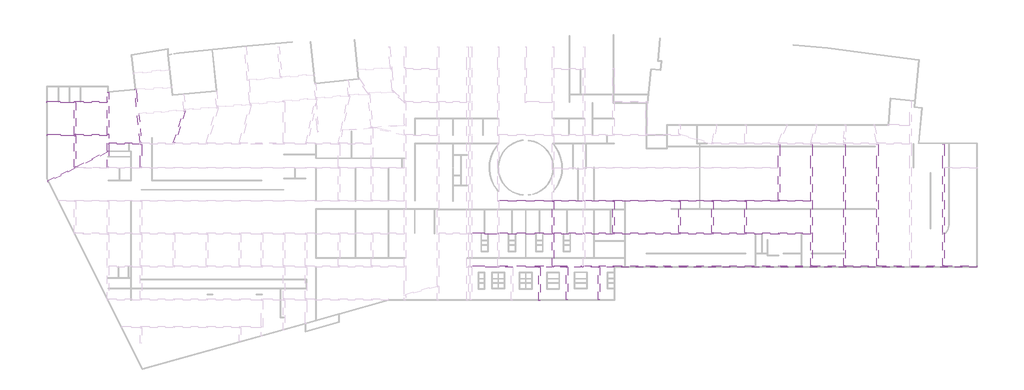
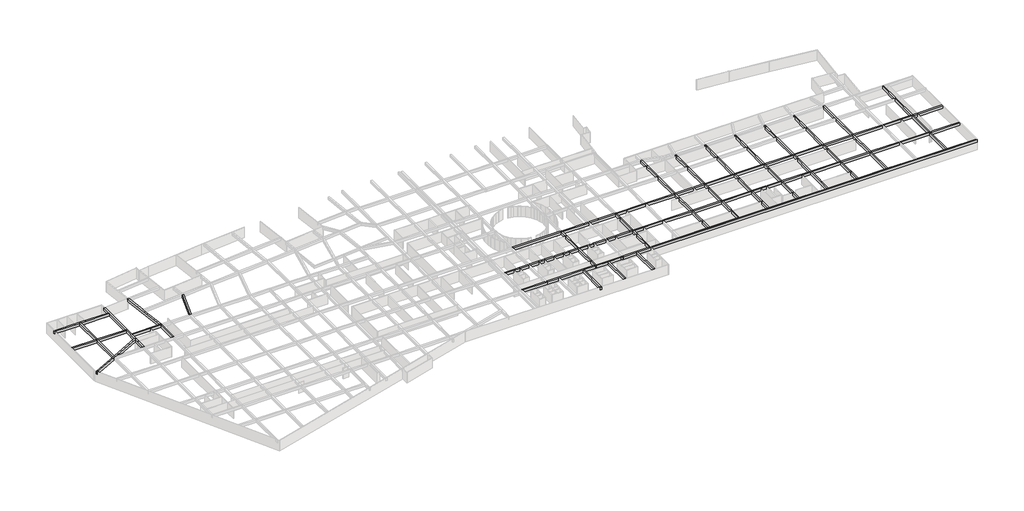
# One storey, part 6 of 8: 38 beams.
"""IFC4 building model written with IfcOpenShell, lengths in millimetres."""

from ifc_helpers import new_model, si_unit, frame, origin, place, context, project, spatial, polyline, outline, extrude, faceted_brep, element, save

model = new_model("IFC4")

# Units and contexts
model_context = context("Model", 3, world=origin())
ifc_project = project(units=[si_unit("LENGTHUNIT", "METRE", prefix="MILLI")], contexts=[model_context])

# Site, building, storey
site = spatial("IfcSite", under=ifc_project)
building = spatial("IfcBuilding", under=site)
storey = spatial("IfcBuildingStorey", under=building, Name="户型图", Elevation=0.0)

# Beams
placement = place(None, origin())
element("IfcBeam", 1, ObjectType="混凝土 - 矩形梁 : KL_beam", at=placement, inside=storey, context=model_context, shape_type="Brep", body=[
    faceted_brep([(544553.8653576, 12938.6264904, 3300.0), (544153.8653576, 12938.6264904, 3300.0), (544153.8653576, 6738.6264904, 3300.0), (544153.8653576, 6338.6264904, 3300.0), (544153.8653576, -2261.3735096, 3300.0), (544153.8653576, -2661.3735096, 3300.0), (544153.8653576, -11261.3735096, 3300.0), (544153.8653576, -11661.3735096, 3300.0), (544153.8653576, -20261.3735096, 3300.0), (544553.8653576, -20261.3735096, 3300.0), (544553.8653576, -11661.3735096, 3300.0), (544553.8653576, -11261.3735096, 3300.0), (544553.8653576, -2661.3735096, 3300.0), (544553.8653576, -2261.3735096, 3300.0), (544553.8653576, 6338.6264904, 3300.0), (544553.8653576, 6738.6264904, 3300.0), (544153.8653576, 12938.6264904, 2500.0), (544153.8653576, 6738.6264904, 2500.0), (544153.8653576, 6338.6264904, 2500.0), (544153.8653576, -2261.3735096, 2500.0), (544153.8653576, -2661.3735096, 2500.0), (544153.8653576, -11261.3735096, 2500.0), (544153.8653576, -11661.3735096, 2500.0), (544153.8653576, -20261.3735096, 2500.0), (544553.8653576, 12938.6264904, 2500.0), (544553.8653576, 6738.6264904, 2500.0), (544553.8653576, 6338.6264904, 2500.0), (544553.8653576, -2261.3735096, 2500.0), (544553.8653576, -2661.3735096, 2500.0), (544553.8653576, -11261.3735096, 2500.0), (544553.8653576, -11661.3735096, 2500.0), (544553.8653576, -20261.3735096, 2500.0)], [[[0, 1, 2, 3, 4, 5, 6, 7, 8, 9, 10, 11, 12, 13, 14, 15]], [[1, 16, 17, 18, 19, 20, 21, 22, 23, 8, 7, 6, 5, 4, 3, 2]], [[16, 24, 25, 26, 27, 28, 29, 30, 31, 23, 22, 21, 20, 19, 18, 17]], [[24, 0, 15, 14, 13, 12, 11, 10, 9, 31, 30, 29, 28, 27, 26, 25]], [[1, 0, 24, 16]], [[9, 8, 23, 31]]]),
])
element("IfcBeam", 2, ObjectType="混凝土 - 矩形梁 : KL_beam", at=placement, inside=storey, context=model_context, shape_type="Brep", body=[
    faceted_brep([(526553.8653576, 12938.6264904, 3300.0), (526153.8653576, 12938.6264904, 3300.0), (526153.8653576, 6738.6264904, 3300.0), (526153.8653576, 6338.6264904, 3300.0), (526153.8653576, -2261.3735096, 3300.0), (526153.8653576, -2661.3735096, 3300.0), (526153.8653576, -11261.3735096, 3300.0), (526153.8653576, -11661.3735096, 3300.0), (526153.8653576, -20261.3735096, 3300.0), (526553.8653576, -20261.3735096, 3300.0), (526553.8653576, -11661.3735096, 3300.0), (526553.8653576, -11261.3735096, 3300.0), (526553.8653576, -2661.3735096, 3300.0), (526553.8653576, -2261.3735096, 3300.0), (526553.8653576, 6338.6264904, 3300.0), (526553.8653576, 6738.6264904, 3300.0), (526153.8653576, 12938.6264904, 2500.0), (526153.8653576, 6738.6264904, 2500.0), (526153.8653576, 6338.6264904, 2500.0), (526153.8653576, -2261.3735096, 2500.0), (526153.8653576, -2661.3735096, 2500.0), (526153.8653576, -11261.3735096, 2500.0), (526153.8653576, -11661.3735096, 2500.0), (526153.8653576, -20261.3735096, 2500.0), (526553.8653576, 12938.6264904, 2500.0), (526553.8653576, 6738.6264904, 2500.0), (526553.8653576, 6338.6264904, 2500.0), (526553.8653576, -2261.3735096, 2500.0), (526553.8653576, -2661.3735096, 2500.0), (526553.8653576, -11261.3735096, 2500.0), (526553.8653576, -11661.3735096, 2500.0), (526553.8653576, -20261.3735096, 2500.0)], [[[0, 1, 2, 3, 4, 5, 6, 7, 8, 9, 10, 11, 12, 13, 14, 15]], [[1, 16, 17, 18, 19, 20, 21, 22, 23, 8, 7, 6, 5, 4, 3, 2]], [[16, 24, 25, 26, 27, 28, 29, 30, 31, 23, 22, 21, 20, 19, 18, 17]], [[24, 0, 15, 14, 13, 12, 11, 10, 9, 31, 30, 29, 28, 27, 26, 25]], [[1, 0, 24, 16]], [[9, 8, 23, 31]]]),
])
element("IfcBeam", 3, ObjectType="混凝土 - 矩形梁 : KL_beam", at=placement, inside=storey, context=model_context, shape_type="Brep", body=[
    faceted_brep([(517553.8653576, 12938.6264904, 3300.0), (517153.8653576, 12938.6264904, 3300.0), (517153.8653576, 6738.6264904, 3300.0), (517153.8653576, 6338.6264904, 3300.0), (517153.8653576, -2261.3735096, 3300.0), (517153.8653576, -2661.3735096, 3300.0), (517153.8653576, -11261.3735096, 3300.0), (517153.8653576, -11661.3735096, 3300.0), (517153.8653576, -20261.3735096, 3300.0), (517553.8653576, -20261.3735096, 3300.0), (517553.8653576, -11661.3735096, 3300.0), (517553.8653576, -11261.3735096, 3300.0), (517553.8653576, -2661.3735096, 3300.0), (517553.8653576, -2261.3735096, 3300.0), (517553.8653576, 6338.6264904, 3300.0), (517553.8653576, 6738.6264904, 3300.0), (517553.8653576, 12938.6264904, 2500.0), (517553.8653576, -20261.3735096, 2500.0), (517553.8653576, -11661.3735096, 2500.0), (517553.8653576, -11261.3735096, 2500.0), (517553.8653576, -2661.3735096, 2500.0), (517553.8653576, -2261.3735096, 2500.0), (517553.8653576, 6338.6264904, 2500.0), (517553.8653576, 6738.6264904, 2500.0), (517153.8653576, 12938.6264904, 2500.0), (517153.8653576, -20261.3735096, 2500.0), (517153.8653576, -11661.3735096, 2500.0), (517153.8653576, -11261.3735096, 2500.0), (517153.8653576, -2661.3735096, 2500.0), (517153.8653576, -2261.3735096, 2500.0), (517153.8653576, 6338.6264904, 2500.0), (517153.8653576, 6738.6264904, 2500.0)], [[[0, 1, 2, 3, 4, 5, 6, 7, 8, 9, 10, 11, 12, 13, 14, 15]], [[16, 0, 15, 14, 13, 12, 11, 10, 9, 17, 18, 19, 20, 21, 22, 23]], [[24, 16, 23, 22, 21, 20, 19, 18, 17, 25, 26, 27, 28, 29, 30, 31]], [[1, 24, 31, 30, 29, 28, 27, 26, 25, 8, 7, 6, 5, 4, 3, 2]], [[1, 0, 16, 24]], [[9, 8, 25, 17]]]),
])
element("IfcBeam", 4, ObjectType="混凝土 - 矩形梁 : KL_beam", at=placement, inside=storey, context=model_context, shape_type="Brep", body=[
    faceted_brep([(508553.8653576, 12938.6264904, 3300.0), (508153.8653576, 12938.6264904, 3300.0), (508153.8653576, 6738.6264904, 3300.0), (508153.8653576, 6338.6264904, 3300.0), (508153.8653576, -2261.3735096, 3300.0), (508153.8653576, -2661.3735096, 3300.0), (508153.8653576, -11261.3735096, 3300.0), (508153.8653576, -11661.3735096, 3300.0), (508153.8653576, -20261.3735096, 3300.0), (508553.8653576, -20261.3735096, 3300.0), (508553.8653576, -11661.3735096, 3300.0), (508553.8653576, -11261.3735096, 3300.0), (508553.8653576, -2661.3735096, 3300.0), (508553.8653576, -2261.3735096, 3300.0), (508553.8653576, 6338.6264904, 3300.0), (508553.8653576, 6738.6264904, 3300.0), (508153.8653576, 12938.6264904, 2500.0), (508153.8653576, 6738.6264904, 2500.0), (508153.8653576, 6338.6264904, 2500.0), (508153.8653576, -2261.3735096, 2500.0), (508153.8653576, -2661.3735096, 2500.0), (508153.8653576, -11261.3735096, 2500.0), (508153.8653576, -11661.3735096, 2500.0), (508153.8653576, -20261.3735096, 2500.0), (508553.8653576, 12938.6264904, 2500.0), (508553.8653576, 6738.6264904, 2500.0), (508553.8653576, 6338.6264904, 2500.0), (508553.8653576, -2261.3735096, 2500.0), (508553.8653576, -2661.3735096, 2500.0), (508553.8653576, -11261.3735096, 2500.0), (508553.8653576, -11661.3735096, 2500.0), (508553.8653576, -20261.3735096, 2500.0)], [[[0, 1, 2, 3, 4, 5, 6, 7, 8, 9, 10, 11, 12, 13, 14, 15]], [[1, 16, 17, 18, 19, 20, 21, 22, 23, 8, 7, 6, 5, 4, 3, 2]], [[16, 24, 25, 26, 27, 28, 29, 30, 31, 23, 22, 21, 20, 19, 18, 17]], [[24, 0, 15, 14, 13, 12, 11, 10, 9, 31, 30, 29, 28, 27, 26, 25]], [[1, 0, 24, 16]], [[9, 8, 23, 31]]]),
])
element("IfcBeam", 5, ObjectType="混凝土 - 矩形梁 : KL_beam", at=placement, inside=storey, context=model_context, shape_type="Brep", body=[
    faceted_brep([(553518.3052108, -2661.3735096, 3300.0), (553518.3052108, -2661.3735096, 2500.0), (553518.3052108, -2261.3735096, 2500.0), (553518.3052108, -2261.3735096, 3300.0), (544553.8653576, -2661.3735096, 3300.0), (544553.8653576, -2261.3735096, 3300.0), (544553.8653576, -2261.3735096, 2500.0), (544553.8653576, -2661.3735096, 2500.0)], [[[0, 1, 2, 3]], [[4, 5, 6, 7]], [[0, 3, 5, 4]], [[3, 2, 6, 5]], [[2, 1, 7, 6]], [[1, 0, 4, 7]]]),
    faceted_brep([(544153.8653576, -2661.3735096, 3300.0), (544153.8653576, -2261.3735096, 3300.0), (535553.8653576, -2261.3735096, 3300.0), (535553.8653576, -2661.3735096, 3300.0), (544153.8653576, -2261.3735096, 2500.0), (535553.8653576, -2261.3735096, 2500.0), (544153.8653576, -2661.3735096, 2500.0), (535553.8653576, -2661.3735096, 2500.0)], [[[0, 1, 2, 3]], [[1, 4, 5, 2]], [[4, 6, 7, 5]], [[6, 0, 3, 7]], [[1, 0, 6, 4]], [[3, 2, 5, 7]]]),
    faceted_brep([(535153.8653576, -2261.3735096, 3300.0), (535153.8653576, -2661.3735096, 3300.0), (535153.8653576, -2661.3735096, 2500.0), (535153.8653576, -2261.3735096, 2500.0), (526553.8653576, -2661.3735096, 3300.0), (526553.8653576, -2261.3735096, 3300.0), (526553.8653576, -2261.3735096, 2500.0), (526553.8653576, -2661.3735096, 2500.0)], [[[0, 1, 2, 3]], [[4, 5, 6, 7]], [[1, 0, 5, 4]], [[0, 3, 6, 5]], [[3, 2, 7, 6]], [[2, 1, 4, 7]]]),
    faceted_brep([(526153.8653576, -2661.3735096, 3300.0), (526153.8653576, -2261.3735096, 3300.0), (517553.8653576, -2261.3735096, 3300.0), (517553.8653576, -2661.3735096, 3300.0), (526153.8653576, -2261.3735096, 2500.0), (517553.8653576, -2261.3735096, 2500.0), (526153.8653576, -2661.3735096, 2500.0), (517553.8653576, -2661.3735096, 2500.0)], [[[0, 1, 2, 3]], [[1, 4, 5, 2]], [[4, 6, 7, 5]], [[6, 0, 3, 7]], [[1, 0, 6, 4]], [[3, 2, 5, 7]]]),
    faceted_brep([(517153.8653576, -2261.3735096, 3300.0), (517153.8653576, -2661.3735096, 3300.0), (517153.8653576, -2661.3735096, 2500.0), (517153.8653576, -2261.3735096, 2500.0), (508553.8653576, -2661.3735096, 3300.0), (508553.8653576, -2261.3735096, 3300.0), (508553.8653576, -2261.3735096, 2500.0), (508553.8653576, -2661.3735096, 2500.0)], [[[0, 1, 2, 3]], [[4, 5, 6, 7]], [[1, 0, 5, 4]], [[0, 3, 6, 5]], [[3, 2, 7, 6]], [[2, 1, 4, 7]]]),
    faceted_brep([(508153.8653576, -2261.3735096, 3300.0), (508153.8653576, -2661.3735096, 3300.0), (508153.8653576, -2661.3735096, 2500.0), (508153.8653576, -2261.3735096, 2500.0), (499653.8653576, -2261.3735096, 3300.0), (499253.8653576, -2261.3735096, 3300.0), (490553.8653576, -2261.3735096, 3300.0), (490153.8653576, -2261.3735096, 3300.0), (481553.8653576, -2261.3735096, 3300.0), (481153.8653576, -2261.3735096, 3300.0), (472553.8653576, -2261.3735096, 3300.0), (472153.8653576, -2261.3735096, 3300.0), (463553.8653576, -2261.3735096, 3300.0), (463153.8653576, -2261.3735096, 3300.0), (454553.8653576, -2261.3735096, 3300.0), (454153.8653576, -2261.3735096, 3300.0), (446453.8653576, -2261.3735096, 3300.0), (446453.8653576, -2661.3735096, 3300.0), (454153.8653576, -2661.3735096, 3300.0), (454553.8653576, -2661.3735096, 3300.0), (463153.8653576, -2661.3735096, 3300.0), (463553.8653576, -2661.3735096, 3300.0), (472153.8653576, -2661.3735096, 3300.0), (472553.8653576, -2661.3735096, 3300.0), (481153.8653576, -2661.3735096, 3300.0), (481553.8653576, -2661.3735096, 3300.0), (490153.8653576, -2661.3735096, 3300.0), (490553.8653576, -2661.3735096, 3300.0), (499253.8653576, -2661.3735096, 3300.0), (499653.8653576, -2661.3735096, 3300.0), (499653.8653576, -2261.3735096, 2500.0), (499253.8653576, -2261.3735096, 2500.0), (490553.8653576, -2261.3735096, 2500.0), (490153.8653576, -2261.3735096, 2500.0), (481553.8653576, -2261.3735096, 2500.0), (481153.8653576, -2261.3735096, 2500.0), (472553.8653576, -2261.3735096, 2500.0), (472153.8653576, -2261.3735096, 2500.0), (463553.8653576, -2261.3735096, 2500.0), (463153.8653576, -2261.3735096, 2500.0), (454553.8653576, -2261.3735096, 2500.0), (454153.8653576, -2261.3735096, 2500.0), (446453.8653576, -2261.3735096, 2500.0), (499653.8653576, -2661.3735096, 2500.0), (499253.8653576, -2661.3735096, 2500.0), (490553.8653576, -2661.3735096, 2500.0), (490153.8653576, -2661.3735096, 2500.0), (481553.8653576, -2661.3735096, 2500.0), (481153.8653576, -2661.3735096, 2500.0), (472553.8653576, -2661.3735096, 2500.0), (472153.8653576, -2661.3735096, 2500.0), (463553.8653576, -2661.3735096, 2500.0), (463153.8653576, -2661.3735096, 2500.0), (454553.8653576, -2661.3735096, 2500.0), (454153.8653576, -2661.3735096, 2500.0), (446453.8653576, -2661.3735096, 2500.0)], [[[0, 1, 2, 3]], [[1, 0, 4, 5, 6, 7, 8, 9, 10, 11, 12, 13, 14, 15, 16, 17, 18, 19, 20, 21, 22, 23, 24, 25, 26, 27, 28, 29]], [[0, 3, 30, 31, 32, 33, 34, 35, 36, 37, 38, 39, 40, 41, 42, 16, 15, 14, 13, 12, 11, 10, 9, 8, 7, 6, 5, 4]], [[3, 2, 43, 44, 45, 46, 47, 48, 49, 50, 51, 52, 53, 54, 55, 42, 41, 40, 39, 38, 37, 36, 35, 34, 33, 32, 31, 30]], [[2, 1, 29, 28, 27, 26, 25, 24, 23, 22, 21, 20, 19, 18, 17, 55, 54, 53, 52, 51, 50, 49, 48, 47, 46, 45, 44, 43]], [[17, 16, 42, 55]]]),
])
element("IfcBeam", 6, ObjectType="混凝土 - 矩形梁 : KL_beam", at=placement, inside=storey, context=model_context, shape_type="Brep", body=[
    faceted_brep([(553518.3052108, -11661.3735096, 3300.0), (553518.3052108, -11661.3735096, 2500.0), (553518.3052108, -11261.3735096, 2500.0), (553518.3052108, -11261.3735096, 3300.0), (544553.8653576, -11661.3735096, 3300.0), (544553.8653576, -11261.3735096, 3300.0), (544553.8653576, -11261.3735096, 2500.0), (544553.8653576, -11661.3735096, 2500.0)], [[[0, 1, 2, 3]], [[4, 5, 6, 7]], [[0, 3, 5, 4]], [[3, 2, 6, 5]], [[2, 1, 7, 6]], [[1, 0, 4, 7]]]),
    faceted_brep([(544153.8653576, -11661.3735096, 3300.0), (544153.8653576, -11261.3735096, 3300.0), (535553.8653576, -11261.3735096, 3300.0), (535553.8653576, -11661.3735096, 3300.0), (544153.8653576, -11261.3735096, 2500.0), (535553.8653576, -11261.3735096, 2500.0), (544153.8653576, -11661.3735096, 2500.0), (535553.8653576, -11661.3735096, 2500.0)], [[[0, 1, 2, 3]], [[1, 4, 5, 2]], [[4, 6, 7, 5]], [[6, 0, 3, 7]], [[1, 0, 6, 4]], [[3, 2, 5, 7]]]),
    faceted_brep([(535153.8653576, -11261.3735096, 3300.0), (535153.8653576, -11661.3735096, 3300.0), (535153.8653576, -11661.3735096, 2500.0), (535153.8653576, -11261.3735096, 2500.0), (526553.8653576, -11661.3735096, 3300.0), (526553.8653576, -11261.3735096, 3300.0), (526553.8653576, -11261.3735096, 2500.0), (526553.8653576, -11661.3735096, 2500.0)], [[[0, 1, 2, 3]], [[4, 5, 6, 7]], [[1, 0, 5, 4]], [[0, 3, 6, 5]], [[3, 2, 7, 6]], [[2, 1, 4, 7]]]),
    faceted_brep([(526153.8653576, -11661.3735096, 3300.0), (526153.8653576, -11261.3735096, 3300.0), (517553.8653576, -11261.3735096, 3300.0), (517553.8653576, -11661.3735096, 3300.0), (526153.8653576, -11261.3735096, 2500.0), (517553.8653576, -11261.3735096, 2500.0), (526153.8653576, -11661.3735096, 2500.0), (517553.8653576, -11661.3735096, 2500.0)], [[[0, 1, 2, 3]], [[1, 4, 5, 2]], [[4, 6, 7, 5]], [[6, 0, 3, 7]], [[1, 0, 6, 4]], [[3, 2, 5, 7]]]),
    faceted_brep([(517153.8653576, -11261.3735096, 3300.0), (517153.8653576, -11661.3735096, 3300.0), (517153.8653576, -11661.3735096, 2500.0), (517153.8653576, -11261.3735096, 2500.0), (508553.8653576, -11661.3735096, 3300.0), (508553.8653576, -11261.3735096, 3300.0), (508553.8653576, -11261.3735096, 2500.0), (508553.8653576, -11661.3735096, 2500.0)], [[[0, 1, 2, 3]], [[4, 5, 6, 7]], [[1, 0, 5, 4]], [[0, 3, 6, 5]], [[3, 2, 7, 6]], [[2, 1, 4, 7]]]),
    faceted_brep([(508153.8653576, -11261.3735096, 3300.0), (508153.8653576, -11661.3735096, 3300.0), (508153.8653576, -11661.3735096, 2500.0), (508153.8653576, -11261.3735096, 2500.0), (499653.8653576, -11261.3735096, 3300.0), (499253.8653576, -11261.3735096, 3300.0), (490553.8653576, -11261.3735096, 3300.0), (490153.8653576, -11261.3735096, 3300.0), (481553.8653576, -11261.3735096, 3300.0), (481153.8653576, -11261.3735096, 3300.0), (472553.8653576, -11261.3735096, 3300.0), (472153.8653576, -11261.3735096, 3300.0), (463553.8653576, -11261.3735096, 3300.0), (463153.8653576, -11261.3735096, 3300.0), (454553.8653576, -11261.3735096, 3300.0), (454153.8653576, -11261.3735096, 3300.0), (446453.8653576, -11261.3735096, 3300.0), (446453.8653576, -11661.3735096, 3300.0), (454153.8653576, -11661.3735096, 3300.0), (454553.8653576, -11661.3735096, 3300.0), (463153.8653576, -11661.3735096, 3300.0), (463553.8653576, -11661.3735096, 3300.0), (472153.8653576, -11661.3735096, 3300.0), (472553.8653576, -11661.3735096, 3300.0), (481153.8653576, -11661.3735096, 3300.0), (481553.8653576, -11661.3735096, 3300.0), (490153.8653576, -11661.3735096, 3300.0), (490553.8653576, -11661.3735096, 3300.0), (499253.8653576, -11661.3735096, 3300.0), (499653.8653576, -11661.3735096, 3300.0), (499653.8653576, -11261.3735096, 2500.0), (499253.8653576, -11261.3735096, 2500.0), (490553.8653576, -11261.3735096, 2500.0), (490153.8653576, -11261.3735096, 2500.0), (481553.8653576, -11261.3735096, 2500.0), (481153.8653576, -11261.3735096, 2500.0), (472553.8653576, -11261.3735096, 2500.0), (472153.8653576, -11261.3735096, 2500.0), (463553.8653576, -11261.3735096, 2500.0), (463153.8653576, -11261.3735096, 2500.0), (454553.8653576, -11261.3735096, 2500.0), (454153.8653576, -11261.3735096, 2500.0), (446453.8653576, -11261.3735096, 2500.0), (499653.8653576, -11661.3735096, 2500.0), (499253.8653576, -11661.3735096, 2500.0), (490553.8653576, -11661.3735096, 2500.0), (490153.8653576, -11661.3735096, 2500.0), (481553.8653576, -11661.3735096, 2500.0), (481153.8653576, -11661.3735096, 2500.0), (472553.8653576, -11661.3735096, 2500.0), (472153.8653576, -11661.3735096, 2500.0), (463553.8653576, -11661.3735096, 2500.0), (463153.8653576, -11661.3735096, 2500.0), (454553.8653576, -11661.3735096, 2500.0), (454153.8653576, -11661.3735096, 2500.0), (446453.8653576, -11661.3735096, 2500.0)], [[[0, 1, 2, 3]], [[1, 0, 4, 5, 6, 7, 8, 9, 10, 11, 12, 13, 14, 15, 16, 17, 18, 19, 20, 21, 22, 23, 24, 25, 26, 27, 28, 29]], [[0, 3, 30, 31, 32, 33, 34, 35, 36, 37, 38, 39, 40, 41, 42, 16, 15, 14, 13, 12, 11, 10, 9, 8, 7, 6, 5, 4]], [[3, 2, 43, 44, 45, 46, 47, 48, 49, 50, 51, 52, 53, 54, 55, 42, 41, 40, 39, 38, 37, 36, 35, 34, 33, 32, 31, 30]], [[2, 1, 29, 28, 27, 26, 25, 24, 23, 22, 21, 20, 19, 18, 17, 55, 54, 53, 52, 51, 50, 49, 48, 47, 46, 45, 44, 43]], [[17, 16, 42, 55]]]),
])
element("IfcBeam", 7, ObjectType="混凝土 - 矩形梁 : KL_beam", at=placement, inside=storey, context=model_context, shape_type="Brep", body=[
    faceted_brep([(553453.8653576, -20261.3735096, 3300.0), (553453.8653576, -20661.3735096, 3300.0), (553453.8653576, -20661.3735096, 2500.0), (553453.8653576, -20261.3735096, 2500.0), (544553.8653576, -20261.3735096, 3300.0), (544153.8653576, -20261.3735096, 3300.0), (535553.8653576, -20261.3735096, 3300.0), (535153.8653576, -20261.3735096, 3300.0), (526553.8653576, -20261.3735096, 3300.0), (526153.8653576, -20261.3735096, 3300.0), (517553.8653576, -20261.3735096, 3300.0), (517153.8653576, -20261.3735096, 3300.0), (508553.8653576, -20261.3735096, 3300.0), (508153.8653576, -20261.3735096, 3300.0), (499653.8653576, -20261.3735096, 3300.0), (499253.8653576, -20261.3735096, 3300.0), (490553.8653576, -20261.3735096, 3300.0), (490153.8653576, -20261.3735096, 3300.0), (481553.8653576, -20261.3735096, 3300.0), (481153.8653576, -20261.3735096, 3300.0), (472553.8653576, -20261.3735096, 3300.0), (472153.8653576, -20261.3735096, 3300.0), (463553.8653576, -20261.3735096, 3300.0), (463153.8653576, -20261.3735096, 3300.0), (454553.8653576, -20261.3735096, 3300.0), (454153.8653576, -20261.3735096, 3300.0), (446453.8653576, -20261.3735096, 3300.0), (446053.8653576, -20261.3735096, 3300.0), (446053.8653576, -20661.3735096, 3300.0), (450103.8653576, -20661.3735096, 3300.0), (450503.8653576, -20661.3735096, 3300.0), (446053.8653576, -20661.3735096, 2500.0), (450103.8653576, -20661.3735096, 2500.0), (450503.8653576, -20661.3735096, 2500.0), (446053.8653576, -20261.3735096, 2500.0), (446453.8653576, -20261.3735096, 2500.0), (454153.8653576, -20261.3735096, 2500.0), (454553.8653576, -20261.3735096, 2500.0), (463153.8653576, -20261.3735096, 2500.0), (463553.8653576, -20261.3735096, 2500.0), (472153.8653576, -20261.3735096, 2500.0), (472553.8653576, -20261.3735096, 2500.0), (481153.8653576, -20261.3735096, 2500.0), (481553.8653576, -20261.3735096, 2500.0), (490153.8653576, -20261.3735096, 2500.0), (490553.8653576, -20261.3735096, 2500.0), (499253.8653576, -20261.3735096, 2500.0), (499653.8653576, -20261.3735096, 2500.0), (508153.8653576, -20261.3735096, 2500.0), (508553.8653576, -20261.3735096, 2500.0), (517153.8653576, -20261.3735096, 2500.0), (517553.8653576, -20261.3735096, 2500.0), (526153.8653576, -20261.3735096, 2500.0), (526553.8653576, -20261.3735096, 2500.0), (535153.8653576, -20261.3735096, 2500.0), (535553.8653576, -20261.3735096, 2500.0), (544153.8653576, -20261.3735096, 2500.0), (544553.8653576, -20261.3735096, 2500.0)], [[[0, 1, 2, 3]], [[1, 0, 4, 5, 6, 7, 8, 9, 10, 11, 12, 13, 14, 15, 16, 17, 18, 19, 20, 21, 22, 23, 24, 25, 26, 27, 28, 29, 30]], [[2, 1, 30, 29, 28, 31, 32, 33]], [[3, 2, 33, 32, 31, 34, 35, 36, 37, 38, 39, 40, 41, 42, 43, 44, 45, 46, 47, 48, 49, 50, 51, 52, 53, 54, 55, 56, 57]], [[0, 3, 57, 56, 55, 54, 53, 52, 51, 50, 49, 48, 47, 46, 45, 44, 43, 42, 41, 40, 39, 38, 37, 36, 35, 34, 27, 26, 25, 24, 23, 22, 21, 20, 19, 18, 17, 16, 15, 14, 13, 12, 11, 10, 9, 8, 7, 6, 5, 4]], [[28, 27, 34, 31]]]),
])
element("IfcBeam", 8, ObjectType="混凝土 - 矩形梁 : KL_beam", at=placement, inside=storey, context=model_context, shape_type="Brep", body=[
    faceted_brep([(472153.8653576, -20261.3735096, 3300.0), (472553.8653576, -20261.3735096, 3300.0), (472553.8653576, -11661.3735096, 3300.0), (472153.8653576, -11661.3735096, 3300.0), (472153.8653576, -20261.3735096, 2500.0), (472153.8653576, -11661.3735096, 2500.0), (472553.8653576, -20261.3735096, 2500.0), (472553.8653576, -11661.3735096, 2500.0)], [[[0, 1, 2, 3]], [[4, 0, 3, 5]], [[6, 4, 5, 7]], [[1, 6, 7, 2]], [[1, 0, 4, 6]], [[3, 2, 7, 5]]]),
    faceted_brep([(472153.8653576, 15338.6264904, 3300.0), (472553.8653576, 15338.6264904, 3300.0), (472553.8653576, 15338.6264904, 2500.0), (472153.8653576, 15338.6264904, 2500.0), (472553.8653576, 6738.6264904, 3300.0), (472153.8653576, 6738.6264904, 3300.0), (472153.8653576, 6738.6264904, 2500.0), (472553.8653576, 6738.6264904, 2500.0), (472553.8653576, 15278.3041611, 3300.0), (472553.8653576, 15278.3041611, 2500.0)], [[[0, 1, 2, 3]], [[4, 5, 6, 7]], [[1, 0, 5, 4, 8]], [[0, 3, 6, 5]], [[3, 2, 9, 7, 6]], [[2, 1, 8, 4, 7, 9]]]),
    faceted_brep([(472553.8653576, -2261.3735096, 3300.0), (472153.8653576, -2261.3735096, 3300.0), (472153.8653576, -2261.3735096, 2500.0), (472553.8653576, -2261.3735096, 2500.0), (472553.8653576, 6338.6264904, 3300.0), (472153.8653576, 6338.6264904, 3300.0), (472153.8653576, 6338.6264904, 2500.0), (472553.8653576, 6338.6264904, 2500.0)], [[[0, 1, 2, 3]], [[1, 0, 4, 5]], [[2, 1, 5, 6]], [[3, 2, 6, 7]], [[0, 3, 7, 4]], [[5, 4, 7, 6]]]),
    faceted_brep([(472153.8653576, -2661.3735096, 3300.0), (472553.8653576, -2661.3735096, 3300.0), (472553.8653576, -2661.3735096, 2500.0), (472153.8653576, -2661.3735096, 2500.0), (472553.8653576, -11261.3735096, 3300.0), (472153.8653576, -11261.3735096, 3300.0), (472153.8653576, -11261.3735096, 2500.0), (472553.8653576, -11261.3735096, 2500.0)], [[[0, 1, 2, 3]], [[4, 5, 6, 7]], [[1, 0, 5, 4]], [[0, 3, 6, 5]], [[3, 2, 7, 6]], [[2, 1, 4, 7]]]),
])
element("IfcBeam", 9, ObjectType="混凝土 - 矩形梁 : KL_beam", at=placement, inside=storey, context=model_context, shape_type="SweptSolid", body=[
    extrude(outline(polyline([(481153.8653576, 12938.6264904), (481553.8653576, 12938.6264904), (481553.8653576, 6738.6264904), (481153.8653576, 6738.6264904), (481153.8653576, 12938.6264904)])), frame((0.0, 0.0, 2500.0), z_axis=(0.0, 0.0, 1.0), x_axis=(1.0, 0.0, 0.0)), (0.0, 0.0, 1.0), 800.0),
    extrude(outline(polyline([(481553.8653576, -20261.3735096), (481153.8653576, -20261.3735096), (481153.8653576, -11661.3735096), (481553.8653576, -11661.3735096), (481553.8653576, -20261.3735096)])), frame((0.0, 0.0, 2500.0), z_axis=(0.0, 0.0, 1.0), x_axis=(1.0, 0.0, 0.0)), (0.0, 0.0, 1.0), 800.0),
    extrude(outline(polyline([(481553.8653576, -2261.3735096), (481153.8653576, -2261.3735096), (481153.8653576, 6338.6264904), (481553.8653576, 6338.6264904), (481553.8653576, -2261.3735096)])), frame((0.0, 0.0, 2500.0), z_axis=(0.0, 0.0, 1.0), x_axis=(1.0, 0.0, 0.0)), (0.0, 0.0, 1.0), 800.0),
    extrude(outline(polyline([(481153.8653576, -2661.3735096), (481553.8653576, -2661.3735096), (481553.8653576, -11261.3735096), (481153.8653576, -11261.3735096), (481153.8653576, -2661.3735096)])), frame((0.0, 0.0, 2500.0), z_axis=(0.0, 0.0, 1.0), x_axis=(1.0, 0.0, 0.0)), (0.0, 0.0, 1.0), 800.0),
])
element("IfcBeam", 10, ObjectType="混凝土 - 矩形梁 : KL_beam", at=placement, inside=storey, context=model_context, shape_type="SweptSolid", body=[
    extrude(outline(polyline([(490553.8653576, -20261.3735096), (490153.8653576, -20261.3735096), (490153.8653576, -11661.3735096), (490553.8653576, -11661.3735096), (490553.8653576, -20261.3735096)])), frame((0.0, 0.0, 2500.0), z_axis=(0.0, 0.0, 1.0), x_axis=(1.0, 0.0, 0.0)), (0.0, 0.0, 1.0), 800.0),
    extrude(outline(polyline([(490153.8653576, 12938.6264904), (490553.8653576, 12938.6264904), (490553.8653576, 6738.6264904), (490153.8653576, 6738.6264904), (490153.8653576, 12938.6264904)])), frame((0.0, 0.0, 2500.0), z_axis=(0.0, 0.0, 1.0), x_axis=(1.0, 0.0, 0.0)), (0.0, 0.0, 1.0), 800.0),
    extrude(outline(polyline([(490553.8653576, -2261.3735096), (490153.8653576, -2261.3735096), (490153.8653576, 6338.6264904), (490553.8653576, 6338.6264904), (490553.8653576, -2261.3735096)])), frame((0.0, 0.0, 2500.0), z_axis=(0.0, 0.0, 1.0), x_axis=(1.0, 0.0, 0.0)), (0.0, 0.0, 1.0), 800.0),
    extrude(outline(polyline([(490153.8653576, -2661.3735096), (490553.8653576, -2661.3735096), (490553.8653576, -11261.3735096), (490153.8653576, -11261.3735096), (490153.8653576, -2661.3735096)])), frame((0.0, 0.0, 2500.0), z_axis=(0.0, 0.0, 1.0), x_axis=(1.0, 0.0, 0.0)), (0.0, 0.0, 1.0), 800.0),
])
element("IfcBeam", 11, ObjectType="混凝土 - 矩形梁 : KL_beam", at=placement, inside=storey, context=model_context, shape_type="Brep", body=[
    faceted_brep([(499653.8653576, 12938.6264904, 3300.0), (499253.8653576, 12938.6264904, 3300.0), (499253.8653576, 6738.6264904, 3300.0), (499253.8653576, 6338.6264904, 3300.0), (499253.8653576, -2261.3735096, 3300.0), (499653.8653576, -2261.3735096, 3300.0), (499653.8653576, 6338.6264904, 3300.0), (499653.8653576, 6738.6264904, 3300.0), (499653.8653576, 12938.6264904, 2500.0), (499653.8653576, -2261.3735096, 2500.0), (499653.8653576, 6338.6264904, 2500.0), (499653.8653576, 6738.6264904, 2500.0), (499253.8653576, 12938.6264904, 2500.0), (499253.8653576, -2261.3735096, 2500.0), (499253.8653576, 6338.6264904, 2500.0), (499253.8653576, 6738.6264904, 2500.0)], [[[0, 1, 2, 3, 4, 5, 6, 7]], [[8, 0, 7, 6, 5, 9, 10, 11]], [[12, 8, 11, 10, 9, 13, 14, 15]], [[1, 12, 15, 14, 13, 4, 3, 2]], [[1, 0, 8, 12]], [[5, 4, 13, 9]]]),
    faceted_brep([(499653.8653576, -20261.3735096, 3300.0), (499253.8653576, -20261.3735096, 3300.0), (499253.8653576, -20261.3735096, 2500.0), (499653.8653576, -20261.3735096, 2500.0), (499253.8653576, -11661.3735096, 3300.0), (499653.8653576, -11661.3735096, 3300.0), (499653.8653576, -11661.3735096, 2500.0), (499253.8653576, -11661.3735096, 2500.0)], [[[0, 1, 2, 3]], [[4, 5, 6, 7]], [[1, 0, 5, 4]], [[0, 3, 6, 5]], [[3, 2, 7, 6]], [[2, 1, 4, 7]]]),
    faceted_brep([(499253.8653576, -2661.3735096, 3300.0), (499653.8653576, -2661.3735096, 3300.0), (499653.8653576, -2661.3735096, 2500.0), (499253.8653576, -2661.3735096, 2500.0), (499253.8653576, -11261.3735096, 3300.0), (499653.8653576, -11261.3735096, 3300.0), (499653.8653576, -11261.3735096, 2500.0), (499253.8653576, -11261.3735096, 2500.0)], [[[0, 1, 2, 3]], [[1, 0, 4, 5]], [[2, 1, 5, 6]], [[3, 2, 6, 7]], [[0, 3, 7, 4]], [[5, 4, 7, 6]]]),
])
element("IfcBeam", 12, ObjectType="混凝土 - 矩形梁 : KL_beam", at=placement, inside=storey, context=model_context, shape_type="SweptSolid", body=[
    extrude(outline(polyline([(454553.8653576, -20261.3735096), (454153.8653576, -20261.3735096), (454153.8653576, -11661.3735096), (454553.8653576, -11661.3735096), (454553.8653576, -20261.3735096)])), frame((0.0, 0.0, 2500.0), z_axis=(0.0, 0.0, 1.0), x_axis=(1.0, 0.0, 0.0)), (0.0, 0.0, 1.0), 800.0),
    extrude(outline(polyline([(454153.8653576, -2661.3735096), (454553.8653576, -2661.3735096), (454553.8653576, -11261.3735096), (454153.8653576, -11261.3735096), (454153.8653576, -2661.3735096)])), frame((0.0, 0.0, 2500.0), z_axis=(0.0, 0.0, 1.0), x_axis=(1.0, 0.0, 0.0)), (0.0, 0.0, 1.0), 800.0),
])
element("IfcBeam", 13, ObjectType="混凝土 - 矩形梁 : KL_beam", at=placement, inside=storey, context=model_context, shape_type="SweptSolid", body=[
    extrude(outline(polyline([(325153.8653576, 12938.6264904), (325553.8653576, 12938.6264904), (325553.8653576, 6738.6264904), (325153.8653576, 6738.6264904), (325153.8653576, 12938.6264904)])), frame((0.0, 0.0, 2500.0), z_axis=(0.0, 0.0, 1.0), x_axis=(1.0, 0.0, 0.0)), (0.0, 0.0, 1.0), 800.0),
])
element("IfcBeam", 14, ObjectType="混凝土 - 矩形梁 : KL_beam", at=placement, inside=storey, context=model_context, shape_type="Brep", body=[
    faceted_brep([(316553.8653576, 15738.6264904, 3300.0), (316153.8653576, 15738.6264904, 3300.0), (316153.8653576, 15338.6264904, 3300.0), (316153.8653576, 11162.2332882, 3300.0), (316153.8653576, 10715.0196927, 3300.0), (316153.8653576, 6738.6264904, 3300.0), (316553.8653576, 6738.6264904, 3300.0), (316553.8653576, 12938.6264904, 3300.0), (316553.8653576, 13338.6264904, 3300.0), (316553.8653576, 15738.6264904, 2500.0), (316553.8653576, 6738.6264904, 2500.0), (316553.8653576, 12938.6264904, 2500.0), (316553.8653576, 13338.6264904, 2500.0), (316153.8653576, 15738.6264904, 2500.0), (316153.8653576, 6738.6264904, 2500.0), (316153.8653576, 10715.0196927, 2500.0), (316153.8653576, 11162.2332882, 2500.0), (316153.8653576, 15338.6264904, 2500.0)], [[[0, 1, 2, 3, 4, 5, 6, 7, 8]], [[9, 0, 8, 7, 6, 10, 11, 12]], [[13, 9, 12, 11, 10, 14, 15, 16, 17]], [[1, 13, 17, 16, 15, 14, 5, 4, 3, 2]], [[6, 5, 14, 10]], [[1, 0, 9, 13]]]),
])
element("IfcBeam", 15, ObjectType="混凝土 - 矩形梁 : KL_beam", at=placement, inside=storey, context=model_context, shape_type="Brep", body=[
    faceted_brep([(307153.8653576, 15738.6264904, 3300.0), (307153.8653576, 15338.6264904, 3300.0), (307553.8653576, 15338.6264904, 3300.0), (316153.8653576, 15338.6264904, 3300.0), (316153.8653576, 15738.6264904, 3300.0), (307553.8653576, 15738.6264904, 3300.0), (307153.8653576, 15738.6264904, 2500.0), (316153.8653576, 15738.6264904, 2500.0), (307553.8653576, 15738.6264904, 2500.0), (307153.8653576, 15338.6264904, 2500.0), (316153.8653576, 15338.6264904, 2500.0), (307553.8653576, 15338.6264904, 2500.0)], [[[0, 1, 2, 3, 4, 5]], [[6, 0, 5, 4, 7, 8]], [[9, 6, 8, 7, 10, 11]], [[1, 9, 11, 10, 3, 2]], [[4, 3, 10, 7]], [[1, 0, 6, 9]]]),
])
element("IfcBeam", 16, ObjectType="混凝土 - 矩形梁 : KL_beam", at=placement, inside=storey, context=model_context, shape_type="Brep", body=[
    faceted_brep([(307553.8653576, 24738.6264904, 3300.0), (307153.8653576, 24738.6264904, 3300.0), (307153.8653576, 24338.6264904, 3300.0), (307153.8653576, 15738.6264904, 3300.0), (307553.8653576, 15738.6264904, 3300.0), (307553.8653576, 24338.6264904, 3300.0), (307553.8653576, 24738.6264904, 2500.0), (307553.8653576, 15738.6264904, 2500.0), (307553.8653576, 24338.6264904, 2500.0), (307153.8653576, 24738.6264904, 2500.0), (307153.8653576, 15738.6264904, 2500.0), (307153.8653576, 24338.6264904, 2500.0)], [[[0, 1, 2, 3, 4, 5]], [[6, 0, 5, 4, 7, 8]], [[9, 6, 8, 7, 10, 11]], [[1, 9, 11, 10, 3, 2]], [[4, 3, 10, 7]], [[1, 0, 6, 9]]]),
])
element("IfcBeam", 17, ObjectType="混凝土 - 矩形梁 : KL_beam", at=placement, inside=storey, context=model_context, shape_type="SweptSolid", body=[
    extrude(outline(polyline([(299553.8653576, 24338.6264904), (299553.8653576, 24738.6264904), (307153.8653576, 24738.6264904), (307153.8653576, 24338.6264904), (299553.8653576, 24338.6264904)])), frame((0.0, 0.0, 2500.0), z_axis=(0.0, 0.0, 1.0), x_axis=(1.0, 0.0, 0.0)), (0.0, 0.0, 1.0), 800.0),
])
element("IfcBeam", 18, ObjectType="混凝土 - 矩形梁 : KL_beam", at=placement, inside=storey, context=model_context, shape_type="SweptSolid", body=[
    extrude(outline(polyline([(299703.8653576, 15338.6264904), (299703.8653576, 15738.6264904), (307153.8653576, 15738.6264904), (307153.8653576, 15338.6264904), (299703.8653576, 15338.6264904)])), frame((0.0, 0.0, 2500.0), z_axis=(0.0, 0.0, 1.0), x_axis=(1.0, 0.0, 0.0)), (0.0, 0.0, 1.0), 800.0),
])
element("IfcBeam", 19, ObjectType="混凝土 - 矩形梁 : KL_beam", at=placement, inside=storey, context=model_context, shape_type="SweptSolid", body=[
    extrude(outline(polyline([(307553.8653576, 24338.6264904), (307553.8653576, 24738.6264904), (316153.8653576, 24738.6264904), (316153.8653576, 24338.6264904), (307553.8653576, 24338.6264904)])), frame((0.0, 0.0, 2500.0), z_axis=(0.0, 0.0, 1.0), x_axis=(1.0, 0.0, 0.0)), (0.0, 0.0, 1.0), 800.0),
])
element("IfcBeam", 20, ObjectType="混凝土 - 矩形梁 : KL_beam", at=placement, inside=storey, context=model_context, shape_type="Brep", body=[
    faceted_brep([(316153.8653576, 27216.9552973, 3300.0), (316553.8653576, 27216.9552973, 3300.0), (316553.8653576, 27216.9552973, 2500.0), (316153.8653576, 27216.9552973, 2500.0), (316153.8653576, 24738.6264904, 3300.0), (316153.8653576, 24338.6264904, 3300.0), (316153.8653576, 15738.6264904, 3300.0), (316553.8653576, 15738.6264904, 3300.0), (316553.8653576, 15738.6264904, 2500.0), (316153.8653576, 15738.6264904, 2500.0), (316153.8653576, 24338.6264904, 2500.0), (316153.8653576, 24738.6264904, 2500.0)], [[[0, 1, 2, 3]], [[1, 0, 4, 5, 6, 7]], [[2, 1, 7, 8]], [[3, 2, 8, 9, 10, 11]], [[0, 3, 11, 10, 9, 6, 5, 4]], [[7, 6, 9, 8]]]),
])
element("IfcBeam", 21, ObjectType="混凝土 - 矩形梁 : KL_beam", at=placement, inside=storey, context=model_context, shape_type="Brep", body=[
    faceted_brep([(299975.0472777, 2625.6106546, 3300.0), (299796.1618395, 2983.381531, 3300.0), (299796.1618395, 2983.381531, 2500.0), (299975.0472777, 2625.6106546, 2500.0), (307153.8653555, 6215.0196927, 3300.0), (307401.078951, 6338.6264904, 3300.0), (308201.0789512, 6738.6264904, 3300.0), (316153.8653576, 10715.0196927, 3300.0), (316153.8653576, 11162.2332882, 3300.0), (307553.8653576, 6862.2332892, 3300.0), (307153.8653576, 6662.2332892, 3300.0), (316153.8653576, 11162.2332882, 2500.0), (307553.8653576, 6862.2332892, 2500.0), (307153.8653576, 6662.2332892, 2500.0), (316153.8653576, 10715.0196927, 2500.0), (308201.0789512, 6738.6264904, 2500.0), (307401.078951, 6338.6264904, 2500.0), (307153.8653555, 6215.0196927, 2500.0)], [[[0, 1, 2, 3]], [[1, 0, 4, 5, 6, 7, 8, 9, 10]], [[2, 1, 10, 9, 8, 11, 12, 13]], [[3, 2, 13, 12, 11, 14, 15, 16, 17]], [[0, 3, 17, 16, 15, 14, 7, 6, 5, 4]], [[8, 7, 14, 11]]]),
])
element("IfcBeam", 22, ObjectType="混凝土 - 矩形梁 : KL_beam", at=placement, inside=storey, context=model_context, shape_type="Brep", body=[
    faceted_brep([(325153.8653576, 12938.6264904, 3300.0), (325153.8653576, 13338.6264904, 3300.0), (325131.7696838, 13338.6264904, 3300.0), (316553.8653576, 13338.6264904, 3300.0), (316553.8653576, 12938.6264904, 3300.0), (325153.8653576, 13338.6264904, 2500.0), (325131.7696838, 13338.6264904, 2500.0), (316553.8653576, 13338.6264904, 2500.0), (325153.8653576, 12938.6264904, 2500.0), (316553.8653576, 12938.6264904, 2500.0)], [[[0, 1, 2, 3, 4]], [[1, 5, 6, 7, 3, 2]], [[5, 8, 9, 7, 6]], [[8, 0, 4, 9]], [[1, 0, 8, 5]], [[4, 3, 7, 9]]]),
])
element("IfcBeam", 23, ObjectType="混凝土 - 矩形梁 : KL_beam", at=placement, inside=storey, context=model_context, shape_type="Brep", body=[
    faceted_brep([(325131.7696838, 13338.6264904, 3300.0), (325153.8653576, 13338.6264904, 3300.0), (325533.9679202, 13338.6264904, 3300.0), (324724.4945588, 21049.1612642, 3300.0), (324682.7246887, 21447.0348091, 3300.0), (324030.1650001, 27662.9085013, 3300.0), (323988.3761227, 28060.9630975, 3300.0), (323590.5623446, 28019.1995019, 3300.0), (325533.9679202, 13338.6264904, 2500.0), (324724.4945588, 21049.1612642, 2500.0), (324682.7246887, 21447.0348091, 2500.0), (324030.1650001, 27662.9085013, 2500.0), (323988.3761227, 28060.9630975, 2500.0), (325153.8653576, 13338.6264904, 2500.0), (325131.7696838, 13338.6264904, 2500.0), (323590.5623446, 28019.1995019, 2500.0)], [[[0, 1, 2, 3, 4, 5, 6, 7]], [[6, 5, 4, 3, 2, 8, 9, 10, 11, 12]], [[12, 11, 10, 9, 8, 13, 14, 15]], [[7, 15, 14, 0]], [[0, 14, 13, 8, 2, 1]], [[7, 6, 12, 15]]]),
])
element("IfcBeam", 24, ObjectType="混凝土 - 矩形梁 : KL_beam", at=placement, inside=storey, context=model_context, shape_type="SweptSolid", body=[
    extrude(outline(polyline([(334626.1752673, 13338.6264904), (334206.9738984, 13338.6264904), (336960.2296074, 22119.6493709), (337391.2547421, 22157.3591839), (334626.1752673, 13338.6264904)])), frame((0.0, 0.0, 2500.0), z_axis=(0.0, 0.0, 1.0), x_axis=(1.0, 0.0, 0.0)), (0.0, 0.0, 1.0), 800.0),
])
element("IfcBeam", 25, ObjectType="混凝土 - 矩形梁 : KL_beam", at=placement, inside=storey, context=model_context, shape_type="SweptSolid", body=[
    extrude(outline(polyline([(307153.8653576, 15338.6264904), (307553.8653576, 15338.6264904), (307553.8653576, 6862.2332892), (307153.8653576, 6662.2332892), (307153.8653576, 15338.6264904)])), frame((0.0, 0.0, 2500.0), z_axis=(0.0, 0.0, 1.0), x_axis=(1.0, 0.0, 0.0)), (0.0, 0.0, 1.0), 800.0),
])
element("IfcBeam", 26, ObjectType="混凝土 - 矩形梁 : KL_beam", at=placement, inside=storey, context=model_context, shape_type="Brep", body=[
    faceted_brep([(437653.8653576, -2261.3735096, 3300.0), (437653.8653576, -2661.3735096, 3300.0), (438053.8653576, -2661.3735096, 3300.0), (446053.8653576, -2661.3735096, 3300.0), (446053.8653576, -2261.3735096, 3300.0), (438053.8653576, -2261.3735096, 3300.0), (437653.8653576, -2261.3735096, 2500.0), (446053.8653576, -2261.3735096, 2500.0), (438053.8653576, -2261.3735096, 2500.0), (437653.8653576, -2661.3735096, 2500.0), (446053.8653576, -2661.3735096, 2500.0), (438053.8653576, -2661.3735096, 2500.0)], [[[0, 1, 2, 3, 4, 5]], [[6, 0, 5, 4, 7, 8]], [[9, 6, 8, 7, 10, 11]], [[1, 9, 11, 10, 3, 2]], [[4, 3, 10, 7]], [[1, 0, 6, 9]]]),
])
element("IfcBeam", 27, ObjectType="混凝土 - 矩形梁 : KL_beam", at=placement, inside=storey, context=model_context, shape_type="SweptSolid", body=[
    extrude(outline(polyline([(437653.8653576, -2261.3735096), (437653.8653576, -2661.3735096), (423053.8653576, -2661.3735096), (423053.8653576, -2261.3735096), (437653.8653576, -2261.3735096)])), frame((0.0, 0.0, 2500.0), z_axis=(0.0, 0.0, 1.0), x_axis=(1.0, 0.0, 0.0)), (0.0, 0.0, 1.0), 800.0),
])
element("IfcBeam", 28, ObjectType="混凝土 - 矩形梁 : KL_beam", at=placement, inside=storey, context=model_context, shape_type="Brep", body=[
    faceted_brep([(437653.8653576, -20661.3735096, 3300.0), (438053.8653576, -20661.3735096, 3300.0), (438053.8653576, -20261.3735096, 3300.0), (438053.8653576, -11661.3735096, 3300.0), (438053.8653576, -11261.3735096, 3300.0), (438053.8653576, -2661.3735096, 3300.0), (437653.8653576, -2661.3735096, 3300.0), (437653.8653576, -11261.3735096, 3300.0), (437653.8653576, -11661.3735096, 3300.0), (437653.8653576, -20261.3735096, 3300.0), (437653.8653576, -20661.3735096, 2500.0), (437653.8653576, -2661.3735096, 2500.0), (437653.8653576, -11261.3735096, 2500.0), (437653.8653576, -11661.3735096, 2500.0), (437653.8653576, -20261.3735096, 2500.0), (438053.8653576, -20661.3735096, 2500.0), (438053.8653576, -2661.3735096, 2500.0), (438053.8653576, -11261.3735096, 2500.0), (438053.8653576, -11661.3735096, 2500.0), (438053.8653576, -20261.3735096, 2500.0)], [[[0, 1, 2, 3, 4, 5, 6, 7, 8, 9]], [[10, 0, 9, 8, 7, 6, 11, 12, 13, 14]], [[15, 10, 14, 13, 12, 11, 16, 17, 18, 19]], [[1, 15, 19, 18, 17, 16, 5, 4, 3, 2]], [[6, 5, 16, 11]], [[1, 0, 10, 15]]]),
])
element("IfcBeam", 29, ObjectType="混凝土 - 矩形梁 : KL_beam", at=placement, inside=storey, context=model_context, shape_type="SweptSolid", body=[
    extrude(outline(polyline([(445353.8653576, -20661.3735096), (445353.8653576, -20261.3735096), (446053.8653576, -20261.3735096), (446053.8653576, -20661.3735096), (445353.8653576, -20661.3735096)])), frame((0.0, 0.0, 2500.0), z_axis=(0.0, 0.0, 1.0), x_axis=(1.0, 0.0, 0.0)), (0.0, 0.0, 1.0), 800.0),
])
element("IfcBeam", 30, ObjectType="混凝土 - 矩形梁 : KL_beam", at=placement, inside=storey, context=model_context, shape_type="Brep", body=[
    faceted_brep([(445353.8653576, -20661.3735096, 3300.0), (445353.8653576, -20261.3735096, 3300.0), (438053.8653576, -20261.3735096, 3300.0), (438053.8653576, -20661.3735096, 3300.0), (441403.8653576, -20661.3735096, 3300.0), (441803.8653576, -20661.3735096, 3300.0), (445353.8653576, -20261.3735096, 2500.0), (438053.8653576, -20261.3735096, 2500.0), (445353.8653576, -20661.3735096, 2500.0), (441803.8653576, -20661.3735096, 2500.0), (441403.8653576, -20661.3735096, 2500.0), (438053.8653576, -20661.3735096, 2500.0)], [[[0, 1, 2, 3, 4, 5]], [[1, 6, 7, 2]], [[6, 8, 9, 10, 11, 7]], [[8, 0, 5, 4, 3, 11, 10, 9]], [[0, 8, 6, 1]], [[3, 2, 7, 11]]]),
])
element("IfcBeam", 31, ObjectType="混凝土 - 矩形梁 : KL_beam", at=placement, inside=storey, context=model_context, shape_type="SweptSolid", body=[
    extrude(outline(polyline([(422653.8653576, -20261.3735096), (422653.8653576, -20460.9013816), (423053.8653576, -20460.9013816), (423053.8653576, -20661.3735096), (415553.8653576, -20661.3735096), (415553.8653576, -20261.3735096), (422653.8653576, -20261.3735096)])), frame((0.0, 0.0, 2500.0), z_axis=(0.0, 0.0, 1.0), x_axis=(1.0, 0.0, 0.0)), (0.0, 0.0, 1.0), 800.0),
])
element("IfcBeam", 32, ObjectType="混凝土 - 矩形梁 : KL_beam", at=placement, inside=storey, context=model_context, shape_type="SweptSolid", body=[
    extrude(outline(polyline([(422653.8653576, -11261.3735096), (422653.8653576, -11661.3735096), (415553.8653576, -11661.3735096), (415553.8653576, -11261.3735096), (422653.8653576, -11261.3735096)])), frame((0.0, 0.0, 2500.0), z_axis=(0.0, 0.0, 1.0), x_axis=(1.0, 0.0, 0.0)), (0.0, 0.0, 1.0), 800.0),
])
element("IfcBeam", 33, ObjectType="混凝土 - 矩形梁 : KL_beam", at=placement, inside=storey, context=model_context, shape_type="SweptSolid", body=[
    extrude(outline(polyline([(446053.8653576, -11261.3735096), (446053.8653576, -11661.3735096), (438053.8653576, -11661.3735096), (438053.8653576, -11261.3735096), (446053.8653576, -11261.3735096)])), frame((0.0, 0.0, 2500.0), z_axis=(0.0, 0.0, 1.0), x_axis=(1.0, 0.0, 0.0)), (0.0, 0.0, 1.0), 800.0),
])
element("IfcBeam", 34, ObjectType="混凝土 - 矩形梁 : KL_beam", at=placement, inside=storey, context=model_context, shape_type="SweptSolid", body=[
    extrude(outline(polyline([(423053.8653576, -11661.3735096), (423053.8653576, -11261.3735096), (437653.8653576, -11261.3735096), (437653.8653576, -11661.3735096), (423053.8653576, -11661.3735096)])), frame((0.0, 0.0, 2500.0), z_axis=(0.0, 0.0, 1.0), x_axis=(1.0, 0.0, 0.0)), (0.0, 0.0, 1.0), 800.0),
])
element("IfcBeam", 35, ObjectType="混凝土 - 矩形梁 : KL_beam", at=placement, inside=storey, context=model_context, shape_type="Brep", body=[
    faceted_brep([(423053.8653576, -20261.3735096, 3300.0), (423053.8653576, -20460.9013816, 3300.0), (423053.8653576, -20661.3735096, 3300.0), (426403.8653576, -20661.3735096, 3300.0), (426803.8653576, -20661.3735096, 3300.0), (433903.8653576, -20661.3735096, 3300.0), (434303.8653576, -20661.3735096, 3300.0), (437653.8653576, -20661.3735096, 3300.0), (437653.8653576, -20261.3735096, 3300.0), (437653.8653576, -20661.3735096, 2500.0), (423053.8653576, -20661.3735096, 2500.0), (426403.8653576, -20661.3735096, 2500.0), (426803.8653576, -20661.3735096, 2500.0), (433903.8653576, -20661.3735096, 2500.0), (434303.8653576, -20661.3735096, 2500.0), (423053.8653576, -20460.9013816, 2500.0), (423053.8653576, -20261.3735096, 2500.0), (437653.8653576, -20261.3735096, 2500.0)], [[[0, 1, 2, 3, 4, 5, 6, 7, 8]], [[9, 7, 6, 5, 4, 3, 2, 10, 11, 12, 13, 14]], [[10, 15, 16, 17, 9, 14, 13, 12, 11]], [[16, 0, 8, 17]], [[0, 16, 15, 10, 2, 1]], [[8, 7, 9, 17]]]),
])
element("IfcBeam", 36, ObjectType="混凝土 - 矩形梁 : KL_beam", at=placement, inside=storey, context=model_context, shape_type="SweptSolid", body=[
    extrude(outline(polyline([(434303.8653576, -29761.3735145), (433903.8653576, -29761.3735145), (433903.8653576, -20661.3735096), (434303.8653576, -20661.3735096), (434303.8653576, -29761.3735145)])), frame((0.0, 0.0, 2500.0), z_axis=(0.0, 0.0, 1.0), x_axis=(1.0, 0.0, 0.0)), (0.0, 0.0, 1.0), 800.0),
])
element("IfcBeam", 37, ObjectType="混凝土 - 矩形梁 : KL_beam", at=placement, inside=storey, context=model_context, shape_type="SweptSolid", body=[
    extrude(outline(polyline([(441803.8653576, -29461.3735145), (441403.8653576, -29461.3735145), (441403.8653576, -20661.3735096), (441803.8653576, -20661.3735096), (441803.8653576, -29461.3735145)])), frame((0.0, 0.0, 2500.0), z_axis=(0.0, 0.0, 1.0), x_axis=(1.0, 0.0, 0.0)), (0.0, 0.0, 1.0), 800.0),
])
element("IfcBeam", 38, ObjectType="混凝土 - 矩形梁 : KL_beam", at=placement, inside=storey, context=model_context, shape_type="SweptSolid", body=[
    extrude(outline(polyline([(450503.8653576, -29461.3735145), (450103.8653576, -29461.3735145), (450103.8653576, -20661.3735096), (450503.8653576, -20661.3735096), (450503.8653576, -29461.3735145)])), frame((0.0, 0.0, 2500.0), z_axis=(0.0, 0.0, 1.0), x_axis=(1.0, 0.0, 0.0)), (0.0, 0.0, 1.0), 800.0),
])

save(model, "model.ifc")

# Revit data of these elements
# Type "混凝土 - 矩形梁 : KL_beam"
#   Length [instance default] = 1524 mm
#   b = 400 mm
#   h = 800 mm
#   Structural Material [instance default] = 混凝土 - 现场浇注混凝土
#   Assembly Code = ""
# Elements 1, 2, 3, 4, 5, 6, 7, 8, 9, 10, 11, 12, 13, 14, 15, 16, 17, 18, 19, 20, 21, 22, 23, 24, 25, 26, 27, 28, 29, 30, 31, 32, 33, 34, 35, 36, 37, 38 (IfcBeam, "混凝土 - 矩形梁 : KL_beam")
#   Comments = ""
#   Structural Material = none
#   Phase Created = 新构造
# Materials
#   "混凝土 - 现场浇注混凝土": class "混凝土", colour RGB 192 192 192, transparency 0
